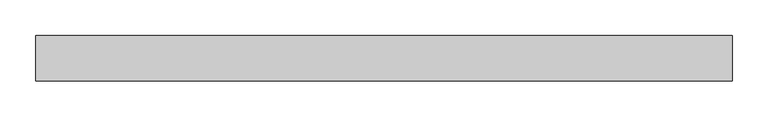
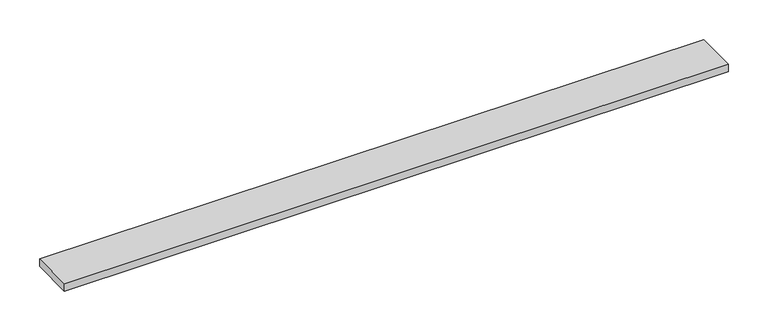
"""IFC4 building model written with IfcOpenShell, lengths in millimetres: proxy geometry, Generic Models 3:Generic Models 1:4:Generic Models 1:4 : Generic Models 3:Generic Models 1:300625:338780:Generic Models 1:4:Generic Models 1:4 : Generic Models 3:Generic Models 1:300625:338780 : Generic Models 3:Generic Models 1:4:Generic Models 1:4 : Generic Models 3:Generic Models 1:300625:338780:4 : Generic Models 3:Generic Models 1:4:Generic Models 1:4 : Generic Models 3:Generic Models 1:300625:338780:Generic Models 1:4:Generic Models 1:4 : Generic Models 3:Generic Models 1:300625:338780 : Generic Models 3:Generic Models 1:4:Generic Models 1:4 : Generic Models 3:Generic Models 1:300625:338780:301383."""

from ifc_helpers import new_model, si_unit, frame, origin, place, context, project, spatial, polyline, outline, extrude, source, transform, mapped, element, save


def generic_models_740093cf(model_context):
    return source(origin(), model_context, "Body", "SweptSolid", [
        extrude(outline(polyline([(593731.7367239, -579032.1885932), (593731.7367239, -579095.3089402), (592761.7742239, -579095.3089402), (592761.7742239, -579032.1885932), (593731.7367239, -579032.1885932)])), frame((0.0, 0.0, 3702.05), z_axis=(0.0, 0.0, 1.0), x_axis=(1.0, 0.0, 0.0)), (0.0, 0.0, 1.0), 11.309767),
    ])


if __name__ == "__main__":
    model = new_model("IFC4")
    model_context = context("Model", 3, world=origin())
    ifc_project = project(units=[si_unit("LENGTHUNIT", "METRE", prefix="MILLI")], contexts=[model_context])
    site = spatial("IfcSite", under=ifc_project)
    building = spatial("IfcBuilding", under=site)
    placement = place(None, origin())
    generic_models_shape = generic_models_740093cf(model_context)
    element("IfcBuildingElementProxy", 1, Name="Generic Models 3:Generic Models 1:4:Generic Models 1:4 : Generic Models 3:Generic Models 1:300625:338780:Generic Models 1:4:Generic Models 1:4 : Generic Models 3:Generic Models 1:300625:338780 : Generic Models 3:Generic Models 1:4:Generic Models 1:4 : Generic Models 3:Generic Models 1:300625:338780:4 : Generic Models 3:Generic Models 1:4:Generic Models 1:4 : Generic Models 3:Generic Models 1:300625:338780:Generic Models 1:4:Generic Models 1:4 : Generic Models 3:Generic Models 1:300625:338780 : Generic Models 3:Generic Models 1:4:Generic Models 1:4 : Generic Models 3:Generic Models 1:300625:338780:301383", ObjectType="Generic Models 3:Generic Models 1:4:Generic Models 1:4 : Generic Models 3:Generic Models 1:300625:338780:Generic Models 1:4:Generic Models 1:4 : Generic Models 3:Generic Models 1:300625:338780 : Generic Models 3:Generic Models 1:4:Generic Models 1:4 : Generic Models 3:Generic Models 1:300625:338780:4 : Generic Models 3:Generic Models 1:4:Generic Models 1:4 : Generic Models 3:Generic Models 1:300625:338780:Generic Models 1:4:Generic Models 1:4 : Generic Models 3:Generic Models 1:300625:338780 : Generic Models 3:Generic Models 1:4:Generic Models 1:4 : Generic Models 3:Generic Models 1:300625:338780:301383", at=placement, inside=building, context=model_context, shape_type="MappedRepresentation", body=[
        mapped(generic_models_shape, transform((0.0, 0.0, 0.0), x_axis=(1.0, 0.0, 0.0), y_axis=(0.0, 1.0, 0.0), z_axis=(0.0, 0.0, 1.0))),
    ])
    save(model, "model.ifc")

# Revit data of these elements
# Type "Generic Models 3:Generic Models 1:4:Generic Models 1:4 : Generic Models 3:Generic Models 1:300625:338780:Generic Models 1:4:Generic Models 1:4 : Generic Models 3:Generic Models 1:300625:338780 : Generic Models 3:Generic Models 1:4:Generic Models 1:4 : Generic Models 3:Generic Models 1:300625:338780:4 : Generic Models 3:Generic Models 1:4:Generic Models 1:4 : Generic Models 3:Generic Models 1:300625:338780:Generic Models 1:4:Generic Models 1:4 : Generic Models 3:Generic Models 1:300625:338780 : Generic Models 3:Generic Models 1:4:Generic Models 1:4 : Generic Models 3:Generic Models 1:300625:338780:301383"
#   NameOverride = "Generic Models 3:Generic Models 1:4:Generic Models 1:4 : Generic Models 3:Generic Models 1:300625:338780:Generic Models 1:4:Generic Models 1:4 : Generic Models 3:Generic Models 1:300625:338780 : Generic Models 3:Generic Models 1:4:Generic Models 1:4 : Generic Models 3:Generic Models 1:300625:338780:301383"
#   ObjectTypeOverride = "Generic Models 1:4:Generic Models 1:4 : Generic Models 3:Generic Models 1:300625:338780 : Generic Models 3:Generic Models 1:4:Generic Models 1:4 : Generic Models 3:Generic Models 1:300625:338780"
#   Reference = "Generic Models 1"
#   Tag = "301383"
# Element 1 (IfcBuildingElementProxy, "Generic Models 3:Generic Models 1:4:Generic Models 1:4 : Generic Models 3:Generic Models 1:300625:338780:Generic Models 1:4:Generic Models 1:4 : Generic Models 3:Generic Models 1:300625:338780 : Generic Models 3:Generic Models 1:4:Generic Models 1:4 : Generic Models 3:Generic Models 1:300625:338780:4 : Generic Models 3:Generic Models 1:4:Generic Models 1:4 : Generic Models 3:Generic Models 1:300625:338780:Generic Models 1:4:Generic Models 1:4 : Generic Models 3:Generic Models 1:300625:338780 : Generic Models 3:Generic Models 1:4:Generic Models 1:4 : Generic Models 3:Generic Models 1:300625:338780:301383")
#   Materials on its faces: "BLOCKING - SIZE AS NEC."
# Materials
#   "BLOCKING - SIZE AS NEC.": class "Wood", colour RGB 144 113 62, transparency 0, Description = "Pinus Echinata", Cost = 0
